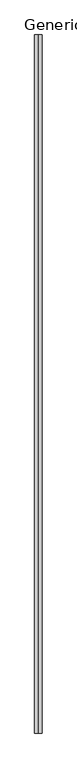
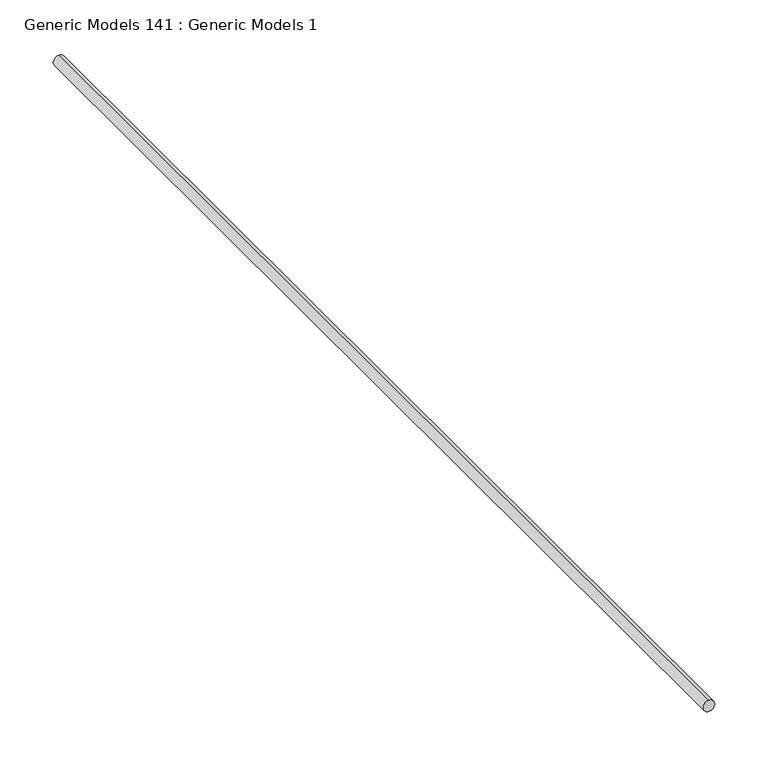
"""IFC4 building model written with IfcOpenShell, lengths in millimetres: proxy geometry, Generic Models 141 : Generic Models 1."""

from ifc_helpers import new_model, si_unit, point, frame, frame_2d, origin, place, context, project, spatial, circle_curve, trimmed, segment, composite_curve, outline, extrude, source, transform, mapped, element, save


def generic_models_141_generic_models_1_a1e14504(model_context):
    return source(origin(), model_context, "Body", "SweptSolid", [
        extrude(outline(composite_curve([segment(trimmed(circle_curve(frame_2d((-554.7288266, 52112.9548165)), 6.35), [point((-548.3788266, 52112.9548165))], [point((-561.0788266, 52112.9548165))], False, "CARTESIAN"), True, "CONTINUOUS"), segment(trimmed(circle_curve(frame_2d((-554.7288266, 52112.9548165)), 6.35), [point((-561.0788266, 52112.9548165))], [point((-548.3788266, 52112.9548165))], False, "CARTESIAN"), True, "CONTINUOUS")], self_intersect=False)), frame((0.0, 0.0, 0.0), z_axis=(0.0, 1.0, 0.0), x_axis=(0.0, 0.0, 1.0)), (0.0, 0.0, 1.0), 1219.2),
    ])


if __name__ == "__main__":
    model = new_model("IFC4")
    model_context = context("Model", 3, world=origin())
    ifc_project = project(units=[si_unit("LENGTHUNIT", "METRE", prefix="MILLI")], contexts=[model_context])
    site = spatial("IfcSite", under=ifc_project)
    building = spatial("IfcBuilding", under=site)
    placement = place(None, origin())
    generic_models_141_generic_models_1_shape = generic_models_141_generic_models_1_a1e14504(model_context)
    element("IfcBuildingElementProxy", 1, Name="Generic Models 141 : Generic Models 1", ObjectType="Generic Models 141 : Generic Models 1", at=placement, inside=building, context=model_context, shape_type="MappedRepresentation", body=[
        mapped(generic_models_141_generic_models_1_shape, transform((0.0, 0.0, 0.0), x_axis=(1.0, 0.0, 0.0), y_axis=(0.0, 1.0, 0.0), z_axis=(0.0, 0.0, 1.0))),
    ])
    save(model, "model.ifc")

# Revit data of these elements
# Element 1 (IfcBuildingElementProxy, "Generic Models 141 : Generic Models 1")
#   Materials on its faces: "#4 CONT. STEEL REBAR"
# Materials
#   "#4 CONT. STEEL REBAR": class "Metal", colour RGB 189 187 185, transparency 0, Description = "Structural steel 50ksi", Cost = 0
